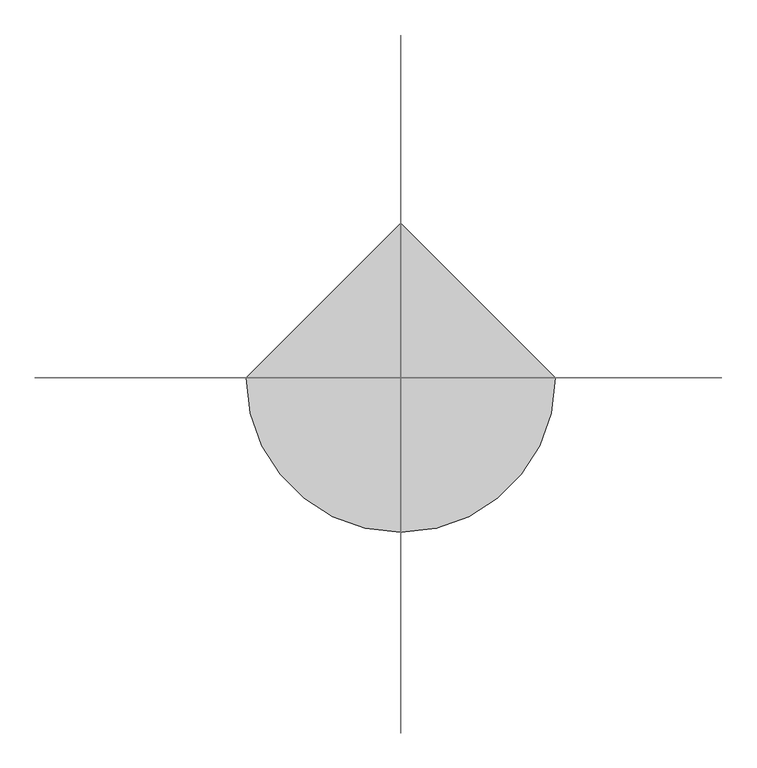
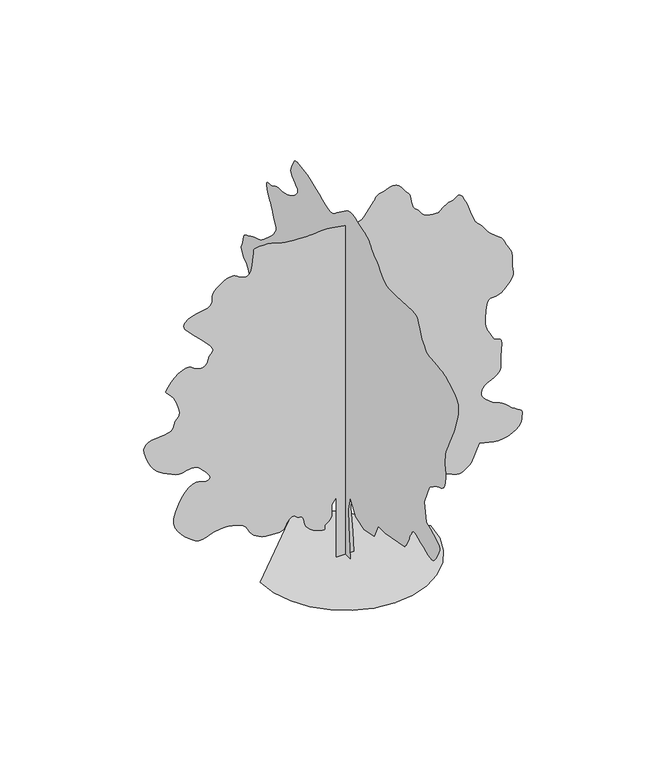
"""IFC4 building model written with IfcOpenShell, lengths in millimetres: geographic element geometry, RPC 木 - 落葉樹 : スカーレット オーク - 12.5 メートル."""

from ifc_helpers import new_model, si_unit, origin, place, context, project, spatial, triangles, source, transform, mapped, element, save


def geographic_element_78a4568a(model_context):
    return source(origin(), model_context, "Body", "Tessellation", [
        triangles([(0.0172504, 306.0074844, 0.0), (0.0172504, -293.5650026, 0.0), (0.0172504, -196.8600042, 1141.1200275), (0.0172504, -177.5185068, 1682.6674953), (0.0172504, -293.5650026, 2185.5350567), (0.0172504, -603.0224945, 1682.6674953), (0.0172504, -1105.8875124, 1527.9400211), (0.0172504, -1686.1174301, 1663.3275421), (0.0172504, -1918.2099495, 2146.8525341), (0.0172504, -2324.3725124, 2146.8525341), (0.0172504, -3446.150116, 2359.6049549), (0.0172504, -3487.4249222, 2409.394939), (0.0172504, -3527.7000801, 2459.5225479), (0.0172504, -3565.9250725, 2510.3249702), (0.0172504, -3601.0999603, 2562.1500046), (0.0172504, -3632.2250954, 2615.3249565), (0.0172504, -3658.2749588, 2670.2000954), (0.0172504, -3678.2499023, 2727.0751122), (0.0172504, -3697.649881, 2785.6750237), (0.0172504, -3722.1251312, 2845.2748741), (0.0172504, -3750.8251236, 2905.7249634), (0.0172504, -3782.89991, 2966.8500114), (0.0172504, -3817.5251221, 3028.475029), (0.0172504, -3853.8249413, 3090.4500252), (0.0172504, -3890.9999977, 3152.5750122), (0.0172504, -3908.7000801, 3172.6499496), (0.0172504, -3933.1750397, 3188.8501236), (0.0172504, -3971.1750458, 3197.2499016), (0.0172504, -4029.4749756, 3193.9751015), (0.0172504, -4114.8499969, 3175.1500877), (0.0172504, -4234.0499886, 3136.8500999), (0.0172504, -4393.8501183, 3075.2250824), (0.0172504, -4562.5749939, 3002.6998581), (0.0172504, -4706.2499451, 2937.9750298), (0.0172504, -4828.2750549, 2886.4249786), (0.0172504, -4932.0251175, 2853.4999535), (0.0172504, -5020.8999252, 2844.5999153), (0.0172504, -5098.249855, 2865.125116), (0.0172504, -5167.5002792, 2920.4999336), (0.0172504, -5237.3750839, 3007.7251328), (0.0172504, -5309.5997452, 3113.9000473), (0.0172504, -5377.1002762, 3229.5499649), (0.0172504, -5432.7497864, 3345.1998825), (0.0172504, -5469.4498718, 3451.3750877), (0.0172504, -5480.1248016, 3538.6249947), (0.0172504, -5457.6250122, 3597.424894), (0.0172504, -5402.6498795, 3641.7000984), (0.0172504, -5323.3000717, 3691.0249947), (0.0172504, -5223.6747574, 3744.5999222), (0.0172504, -5107.774855, 3801.5499344), (0.0172504, -4979.7251129, 3861.0500816), (0.0172504, -4843.5499947, 3922.2251266), (0.0172504, -4703.3251236, 3984.2501198), (0.0172504, -4587.2749397, 4641.8500969), (0.0172504, -4877.3749649, 5318.7747665), (0.0172504, -4886.5249878, 5331.7001404), (0.0172504, -4900.7252838, 5347.4747589), (0.0172504, -4925.0999588, 5369.0251877), (0.0172504, -4964.6748688, 5399.20009), (0.0172504, -5024.5502838, 5440.8498734), (0.0172504, -5109.8247299, 5496.8999405), (0.0172504, -5225.5252258, 5570.225116), (0.0172504, -5351.0501221, 5636.6501312), (0.0172504, -5462.3497238, 5680.0498077), (0.0172504, -5559.4501923, 5715.3499786), (0.0172504, -5642.3497833, 5757.424736), (0.0172504, -5711.0252426, 5821.1499161), (0.0172504, -5765.4998245, 5921.4001923), (0.0172504, -5805.7502747, 6073.0752365), (0.0172504, -5829.0500153, 6222.0498642), (0.0172504, -5835.7501877, 6317.5748474), (0.0172504, -5830.6249191, 6379.6001312), (0.0172504, -5818.3750854, 6428.1000778), (0.0172504, -5803.7748138, 6483.0252136), (0.0172504, -5791.5499786, 6564.3249023), (0.0172504, -5786.4247101, 6692.0002487), (0.0172504, -5788.2251816, 6832.849791), (0.0172504, -5796.1252808, 6949.6752182), (0.0172504, -5813.8247818, 7056.3751007), (0.0172504, -5845.0502014, 7166.7747574), (0.0172504, -5893.550148, 7294.7750839), (0.0172504, -5963.0249771, 7454.2502335), (0.0172504, -6057.1750443, 7659.049942), (0.0172504, -6146.5748199, 7844.1752701), (0.0172504, -6206.1752518, 7955.8748474), (0.0172504, -6246.4751175, 8024.9502823), (0.0172504, -6277.9999374, 8082.1752777), (0.0172504, -6311.225235, 8158.3502792), (0.0172504, -6356.599791, 8284.2751511), (0.0172504, -6424.6752869, 8490.6997604), (0.0172504, -6498.0248795, 8729.4997192), (0.0172504, -6547.3747742, 8935.1499573), (0.0172504, -6565.2498459, 9112.3751862), (0.0172504, -6544.199968, 9265.925116), (0.0172504, -6476.8250107, 9400.5250397), (0.0172504, -6355.6498489, 9520.9002502), (0.0172504, -6173.2249374, 9631.8248749), (0.0172504, -5996.2252762, 9723.0001236), (0.0172504, -5879.7998245, 9785.7747803), (0.0172504, -5799.2250916, 9827.2001587), (0.0172504, -5729.8002594, 9854.4496582), (0.0172504, -5646.85009, 9874.575174), (0.0172504, -5525.6749283, 9894.699527), (0.0172504, -5341.575119, 9921.9501892), (0.0172504, -5144.0999634, 9943.4244598), (0.0172504, -4990.9500092, 9951.725116), (0.0172504, -4869.5998581, 9962.0244873), (0.0172504, -4767.5499825, 9989.5995483), (0.0172504, -4672.2499855, 10049.6505341), (0.0172504, -4571.2000488, 10157.425351), (0.0172504, -4451.8750648, 10328.0998169), (0.0172504, -4347.6750298, 10515.7499908), (0.0172504, -4286.1000092, 10666.5500885), (0.0172504, -4245.8501404, 10783.8254883), (0.0172504, -4205.5749825, 10871.0003998), (0.0172504, -4143.9999619, 10931.4501984), (0.0172504, -4039.7999268, 10968.5502594), (0.0172504, -3871.650016, 10985.7003754), (0.0172504, -2943.2749969, 10927.6748474), (0.0172504, -2772.1499771, 10930.6746643), (0.0172504, -2632.8250511, 10930.2746887), (0.0172504, -2514.4500092, 10937.3254211), (0.0172504, -2406.244986, 10962.6250397), (0.0172504, -2297.3600624, 11017.0496246), (0.0172504, -2176.9724979, 11111.3752625), (0.0172504, -2034.2550465, 11256.4745453), (0.0172504, -1896.7275398, 11403.0249023), (0.0172504, -1793.7050491, 11502.8746216), (0.0172504, -1717.0749882, 11568.5752625), (0.0172504, -1658.7125622, 11612.6248993), (0.0172504, -1610.5025688, 11647.5250946), (0.0172504, -1564.320068, 11685.7995026), (0.0172504, -1512.0500027, 11739.9996826), (0.0172504, -1461.8649845, 11804.0004272), (0.0172504, -1420.8125484, 11863.6002777), (0.0172504, -1379.087479, 11919.1503754), (0.0172504, -1326.8724976, 11970.9495392), (0.0172504, -1254.3574471, 12019.4000702), (0.0172504, -1151.7299904, 12064.7996246), (0.0172504, -1009.182514, 12107.4749268), (0.0172504, -849.1549999, 12154.4999634), (0.0172504, -699.9524792, 12206.6002716), (0.0172504, -560.5600064, 12254.6496643), (0.0172504, -429.9675053, 12289.4998627), (0.0172504, -307.1550161, 12302.0246796), (0.0172504, -191.1079934, 12283.0746735), (0.0172504, -80.8134993, 12223.5248199), (0.0172504, 499.4175176, 11798.0252106), (0.0172504, 562.2325061, 11740.8496307), (0.0172504, 623.0199657, 11688.7504852), (0.0172504, 689.217524, 11646.7751404), (0.0172504, 768.2749804, 11620.0500275), (0.0172504, 867.630035, 11613.6248383), (0.0172504, 994.7275097, 11632.5748444), (0.0172504, 1157.0125168, 11681.9753174), (0.0172504, 1341.1749676, 11755.3254913), (0.0172504, 1526.6899521, 11837.8251068), (0.0172504, 1710.1749733, 11922.0246185), (0.0172504, 1888.2475342, 12000.4500641), (0.0172504, 2057.5249924, 12065.6995697), (0.0172504, 2214.6200546, 12110.3003357), (0.0172504, 2356.1550201, 12126.8249084), (0.0172504, 2484.8875694, 12135.849939), (0.0172504, 2604.4750374, 12156.3754303), (0.0172504, 2712.9251038, 12178.575238), (0.0172504, 2808.1501053, 12192.6755402), (0.0172504, 2888.1748718, 12188.8501923), (0.0172504, 2950.9251114, 12157.2753754), (0.0172504, 2994.400074, 12088.1249451), (0.0172504, 3033.2500282, 12001.2500153), (0.0172504, 3077.8499222, 11921.1246735), (0.0172504, 3119.7499809, 11845.0502472), (0.0172504, 3150.5001389, 11770.3245758), (0.0172504, 3161.6000427, 11694.2745667), (0.0172504, 3144.6249161, 11614.1503876), (0.0172504, 3091.124984, 11527.2498779), (0.0172504, 3009.2500397, 11447.6245056), (0.0172504, 2921.5998665, 11385.2504059), (0.0172504, 2841.4251091, 11331.3502075), (0.0172504, 2781.8749649, 11277.1000305), (0.0172504, 2756.1750801, 11213.7248291), (0.0172504, 2777.4749428, 11132.4251404), (0.0172504, 2859.0249069, 11024.3747589), (0.0172504, 2971.6250107, 10916.7255157), (0.0172504, 3077.7999252, 10838.2000763), (0.0172504, 3178.2249001, 10782.3), (0.0172504, 3273.574894, 10742.6745117), (0.0172504, 3364.5248657, 10712.8251709), (0.0172504, 3451.7750633, 10686.4000397), (0.0172504, 3535.9498672, 10656.8995148), (0.0172504, 3620.024968, 10634.1753204), (0.0172504, 3706.4749237, 10626.6746155), (0.0172504, 3795.2750267, 10625.9502411), (0.0172504, 3886.4499847, 10623.5248077), (0.0172504, 3980.0000885, 10610.9499939), (0.0172504, 4075.9250473, 10579.7495728), (0.0172504, 4174.1998627, 10521.5252197), (0.0172504, 4275.775058, 10469.80047), (0.0172504, 4375.6250679, 10451.2504395), (0.0172504, 4465.0001358, 10446.8995422), (0.0172504, 4535.0999268, 10437.8245148), (0.0172504, 4577.0999794, 10405.075351), (0.0172504, 4582.2249573, 10329.6753021), (0.0172504, 4541.7001053, 10192.7255219), (0.0172504, 4481.7999825, 10048.5994354), (0.0172504, 4432.0751106, 9951.4995483), (0.0172504, 4388.424868, 9882.1247131), (0.0172504, 4346.8250816, 9821.224942), (0.0172504, 4303.1751297, 9749.5002502), (0.0172504, 4253.4249687, 9647.6750702), (0.0172504, 4193.550135, 9496.4499985), (0.0172504, 4130.2749275, 9347.6997757), (0.0172504, 4075.8250534, 9253.7502777), (0.0172504, 4034.1999779, 9195.999733), (0.0172504, 4009.500032, 9155.8498581), (0.0172504, 4005.7749687, 9114.7000443), (0.0172504, 4027.1001205, 9053.900267), (0.0172504, 4077.4999512, 8954.8999146), (0.0172504, 4167.2249977, 8823.6747849), (0.0172504, 4293.1248711, 8684.3501495), (0.0172504, 4439.3499573, 8545.349913), (0.0172504, 4589.9500671, 8415.1497208), (0.0172504, 4729.0750053, 8302.2002197), (0.0172504, 4840.7748734, 8214.9747299), (0.0172504, 4909.1747681, 8161.9000626), (0.0172504, 4969.9001312, 8128.6997635), (0.0172504, 5061.0747986, 8095.1500671), (0.0172504, 5170.5250946, 8060.9248306), (0.0172504, 5286.0750183, 8025.675238), (0.0172504, 5395.524733, 7989.0751465), (0.0172504, 5486.6999817, 7950.8001572), (0.0172504, 5547.4247635, 7910.4747116), (0.0172504, 5598.275148, 7876.9750122), (0.0172504, 5663.0252655, 7853.2997131), (0.0172504, 5734.1749924, 7830.2999542), (0.0172504, 5804.3247803, 7798.8251312), (0.0172504, 5866.0250839, 7749.7752182), (0.0172504, 5911.8001968, 7673.9751938), (0.0172504, 5934.2499893, 7562.325032), (0.0172504, 5952.6250305, 7450.1749008), (0.0172504, 5984.1998474, 7370.8500916), (0.0172504, 6018.4750809, 7312.1501862), (0.0172504, 6045.000206, 7261.899765), (0.0172504, 6053.2252853, 7207.9501511), (0.0172504, 6032.699794, 7138.074765), (0.0172504, 5972.9249542, 7040.1249298), (0.0172504, 5898.7248322, 6948.3747162), (0.0172504, 5838.7250061, 6893.5251572), (0.0172504, 5788.2001831, 6857.9500031), (0.0172504, 5742.4000717, 6824.0497467), (0.0172504, 5696.6249588, 6774.2498795), (0.0172504, 5646.1001358, 6690.9747299), (0.0172504, 5586.0997284, 6556.5997925), (0.0172504, 5520.7002319, 6421.9998688), (0.0172504, 5460.6998245, 6337.1498154), (0.0172504, 5411.5249191, 6283.075209), (0.0172504, 5378.6001846, 6240.824881), (0.0172504, 5367.3247101, 6191.4999847), (0.0172504, 5383.09991, 6116.0999359), (0.0172504, 5431.3748703, 5995.7247253), (0.0172504, 5495.5000259, 5864.0502045), (0.0172504, 5555.8748291, 5761.8250488), (0.0172504, 5613.5747955, 5680.5747757), (0.0172504, 5669.5498672, 5611.8249023), (0.0172504, 5724.8749786, 5547.1497803), (0.0172504, 5780.5250702, 5478.0749268), (0.0172504, 5837.5250793, 5396.1502762), (0.0172504, 5903.6751114, 5315.3499756), (0.0172504, 5980.6500641, 5249.4249298), (0.0172504, 6060.324852, 5189.6000931), (0.0172504, 6134.5999695, 5127.0498413), (0.0172504, 6195.3247513, 5053.0252899), (0.0172504, 6234.4002731, 4958.675235), (0.0172504, 6243.7002869, 4835.2499199), (0.0172504, 6251.5248093, 4738.3250221), (0.0172504, 6280.349794, 4706.349939), (0.0172504, 6313.2251129, 4704.825032), (0.0172504, 6333.2500534, 4699.2500816), (0.0172504, 6323.4750687, 4655.0998695), (0.0172504, 6267.0500244, 4537.8750481), (0.0172504, 6146.999794, 4313.0501083), (0.0172504, 6021.4748978, 4060.8750938), (0.0172504, 5945.6998718, 3875.3750793), (0.0172504, 5898.3248566, 3742.6250427), (0.0172504, 5858.0749878, 3648.7999557), (0.0172504, 5803.5998245, 3580.0000854), (0.0172504, 5713.6000854, 3522.3751144), (0.0172504, 5566.7747452, 3462.0500175), (0.0172504, 5397.250209, 3413.1000984), (0.0172504, 5248.0500137, 3392.5748978), (0.0172504, 5111.025238, 3390.9999939), (0.0172504, 4978.0752136, 3398.9000931), (0.0172504, 4841.0498566, 3406.7749031), (0.0172504, 4691.8499519, 3405.1999992), (0.0172504, 4522.3501236, 3384.6750893), (0.0172504, 4353.2999771, 3366.3000481), (0.0172504, 4207.2498802, 3370.2500977), (0.0172504, 4078.7998718, 3385.7000267), (0.0172504, 3962.5249924, 3401.8249146), (0.0172504, 3853.0249901, 3407.8001312), (0.0172504, 3744.8749054, 3392.799884), (0.0172504, 3632.6500694, 3346.0001244), (0.0172504, 3525.249939, 3296.2499634), (0.0172504, 3436.4251282, 3270.2000999), (0.0172504, 3368.249929, 3253.6249489), (0.0172504, 3322.75009, 3232.3250862), (0.0172504, 3301.9499062, 3192.0499283), (0.0172504, 3307.8751259, 3118.6500481), (0.0172504, 3342.5500443, 2997.8498634), (0.0172504, 3398.475119, 2869.5251381), (0.0172504, 3465.5750931, 2778.7248665), (0.0172504, 3542.0000793, 2719.2500084), (0.0172504, 3625.8499031, 2684.8000763), (0.0172504, 3715.274968, 2669.1248703), (0.0172504, 3808.4250961, 2665.9500641), (0.0172504, 3903.4251114, 2669.0498749), (0.0172504, 4270.9250633, 2262.8999565), (0.0172504, 4299.7250496, 2217.1674282), (0.0172504, 4327.3501076, 2170.5925095), (0.0172504, 4352.6250183, 2122.3249615), (0.0172504, 4374.3248566, 2071.5174522), (0.0172504, 4391.2999832, 2017.3300621), (0.0172504, 4402.3498901, 1958.9125523), (0.0172504, 4406.2999397, 1895.4200615), (0.0172504, 4405.6249809, 1829.2200325), (0.0172504, 4400.8999786, 1763.6974331), (0.0172504, 4388.0248924, 1699.5299835), (0.0172504, 4362.9999664, 1637.3900265), (0.0172504, 4321.7248695, 1577.9574623), (0.0172504, 4260.1501396, 1521.9075405), (0.0172504, 4174.1998627, 1469.9175453), (0.0172504, 4092.2249245, 1425.7650078), (0.0172504, 4034.5999535, 1391.4249527), (0.0172504, 3985.4250481, 1364.8675621), (0.0172504, 3928.800016, 1344.0599659), (0.0172504, 3848.8499542, 1326.9749622), (0.0172504, 3729.6499626, 1311.5799717), (0.0172504, 3555.3001396, 1295.8475018), (0.0172504, 3356.9750359, 1298.1024513), (0.0172504, 3174.2251442, 1332.8375404), (0.0172504, 3003.6500908, 1392.27243), (0.0172504, 2841.8750816, 1468.6199501), (0.0172504, 2685.525032, 1554.1049938), (0.0172504, 2531.1748604, 1640.9425713), (0.0172504, 2375.4949734, 1721.3500179), (0.0172504, 2236.6675461, 1794.4849434), (0.0172504, 2129.3050587, 1863.5599422), (0.0172504, 2044.6099377, 1926.8850014), (0.0172504, 1973.7875164, 1982.7650208), (0.0172504, 1908.0399307, 2029.5099873), (0.0172504, 1838.5700432, 2065.4300331), (0.0172504, 1756.5824604, 2088.8300583), (0.0172504, 1666.4174698, 2108.5650455), (0.0172504, 1577.6074837, 2133.0375343), (0.0172504, 1489.134977, 2159.8799366), (0.0172504, 1399.9875114, 2186.7200134), (0.0172504, 1309.1449459, 2211.1925022), (0.0172504, 1215.5975309, 2230.9274895), (0.0172504, 1118.3299942, 2243.5575325), (0.0172504, 1018.8625191, 2250.1549496), (0.0172504, 919.3925005, 2253.7074944), (0.0172504, 819.9250254, 2254.7225487), (0.0172504, 720.4574776, 2253.7074944), (0.0172504, 620.9900024, 2251.1700039), (0.0172504, 521.5199839, 2247.6174591), (0.0172504, 422.0525087, 2243.5575325), (0.0172504, 228.6430025, 1953.4425373), (0.0172504, 189.960498, 1508.6000679), (280.4450004, 0.0006008, 0.0092122), (-299.7850081, 0.0006008, 0.0092122), (-299.7850081, 0.0004756, 2127.5199932), (-454.5149895, 0.0004756, 1914.7700432), (-454.5149895, 0.0005007, 1682.6775238), (-450.9625174, 0.0005007, 1628.8274677), (-450.9625174, 0.0005007, 1575.1449886), (-458.0674979, 0.0005007, 1521.8024597), (-475.8274967, 0.0005257, 1468.967458), (-507.8000001, 0.0005257, 1416.8100311), (-557.5350094, 0.0005257, 1365.4949947), (-628.5824896, 0.0005257, 1315.1974834), (-684.2375227, 0.0005257, 1262.982502), (-699.6325132, 0.0005257, 1210.0900183), (-696.0799685, 0.0005257, 1162.9524885), (-694.8950117, 0.0005257, 1127.990015), (-717.3950191, 0.0005257, 1111.6375248), (-784.8900272, 0.0005257, 1120.3225325), (-918.6974848, 0.0005257, 1160.4700092), (-1071.3399845, 0.0005257, 1223.0050003), (-1185.4125275, 0.0005257, 1293.6575191), (-1267.3425556, 0.0005257, 1371.0799736), (-1323.5625252, 0.0005257, 1453.9125629), (-1360.49748, 0.0005007, 1540.8049335), (-1384.5749348, 0.0005007, 1630.4049877), (-1402.2250202, 0.0005007, 1721.3600464), (-1406.7350647, 0.0005007, 1746.1124599), (-1413.4449749, 0.0005007, 1770.19006), (-1424.5524364, 0.0005007, 1792.9174519), (-1442.2599312, 0.0005007, 1813.6099388), (-1468.7600578, 0.0005007, 1831.5975037), (-1506.2599491, 0.0005007, 1846.2025715), (-1556.9524944, 0.0005007, 1856.7475674), (-1607.6450397, 0.0005007, 1874.1124958), (-1647.5100483, 0.0005007, 1903.3224861), (-1682.3025467, 0.0004756, 1934.9000645), (-1717.7700039, 0.0004756, 1959.3725533), (-1759.6674465, 0.0004756, 1967.2675655), (-1813.7424889, 0.0004756, 1949.1099529), (-1885.7500122, 0.0005007, 1895.4274738), (-1949.0724552, 0.0005007, 1820.3199944), (-1984.9925011, 0.0005007, 1746.902528), (-2011.1000645, 0.0005007, 1679.2374722), (-2044.9875309, 0.0005007, 1621.382428), (-2104.2525181, 0.0005007, 1577.4025543), (-2206.4824699, 0.0005007, 1551.3499294), (-2369.2750042, 0.0005007, 1547.2900028), (-2549.149926, 0.0005007, 1559.2449417), (-2695.2000229, 0.0005007, 1578.979929), (-2813.8250496, 0.0005007, 1607.1750103), (-2911.4999016, 0.0005007, 1644.5025284), (-2994.6250603, 0.0005007, 1691.6425289), (-3069.600135, 0.0005007, 1749.2724415), (-3142.9250198, 0.0005007, 1818.0650448), (-3205.1000038, 0.0005007, 1893.5100037), (-3249.7248962, 0.0004756, 1969.2975288), (-3287.549913, 0.0004756, 2043.389954), (-3329.4499718, 0.0004756, 2113.7625481), (-3386.2249947, 0.0004756, 2178.3824409), (-3468.7249008, 0.0004756, 2235.2224308), (-3587.7499031, 0.0004756, 2282.2499382), (-3707.4248657, 0.0004756, 2317.9974655), (-3794.2500893, 0.0004506, 2343.2600224), (-3862.8249733, 0.0004506, 2359.3875263), (-3927.6750847, 0.0004506, 2367.7325111), (-4003.3251183, 0.0004506, 2369.6499813), (-4104.3750549, 0.0004506, 2366.4924706), (-4245.3498802, 0.0004506, 2359.6125126), (-4400.3500122, 0.0004506, 2335.1974331), (-4538.1250328, 0.0004756, 2289.8050003), (-4665.0501343, 0.0004756, 2240.3524956), (-4787.5749229, 0.0004756, 2203.7574909), (-4912.1501678, 0.0004756, 2196.9349422), (-5045.1501892, 0.0004756, 2236.7999508), (-5193.0498825, 0.0004506, 2340.2725594), (-5347.7997391, 0.0004506, 2478.6475433), (-5490.6747391, 0.0004506, 2615.9999153), (-5612.2498764, 0.0004256, 2758.4499413), (-5703.0251495, 0.0004256, 2912.049868), (-5753.5499725, 0.0004256, 3082.8999046), (-5754.3499237, 0.0004005, 3277.0999695), (-5695.9250015, 0.0004005, 3500.7249825), (-5598.1501556, 0.0003755, 3726.2748779), (-5489.1998291, 0.0003755, 3919.6999901), (-5372.1499969, 0.0003505, 4077.2499664), (-5250.0248932, 0.0003505, 4195.2000343), (-5125.8499146, 0.0003505, 4269.8501289), (-5002.6998734, 0.0003505, 4297.4998947), (-4883.6001663, 0.0003505, 4274.3751434), (-4771.2750458, 0.0003505, 4235.4749016), (-4671.8250114, 0.0003505, 4218.8750427), (-4593.3248611, 0.0003505, 4225.6499199), (-4543.9249695, 0.0003505, 4256.7750549), (-4531.7501312, 0.0003505, 4313.2750946), (-4564.9001427, 0.0003505, 4396.1749763), (-4651.5000893, 0.0003254, 4506.4749298), (-4752.500029, 0.0003254, 4617.0998634), (-4829.4749817, 0.0003254, 4702.3498924), (-4891.5502625, 0.0003254, 4765.2751213), (-4947.8747314, 0.0003254, 4808.9250732), (-5007.6001556, 0.0003254, 4836.325145), (-5079.8248169, 0.0003004, 4850.5498581), (-5173.7248993, 0.0003004, 4854.5999016), (-5270.0248352, 0.0003254, 4845.5248741), (-5349.7751999, 0.0003254, 4824.5999886), (-5422.3998367, 0.0003254, 4801.3249557), (-5497.39991, 0.0003254, 4785.1250725), (-5584.2248428, 0.0003254, 4785.5250481), (-5692.3752182, 0.0003254, 4811.9748871), (-5831.3248764, 0.0003004, 4873.9498833), (-5978.7751785, 0.0003004, 4948.0997177), (-6108.6248108, 0.0003004, 5012.4248611), (-6224.6252884, 0.0003004, 5078.4748993), (-6330.4502243, 0.0003004, 5157.6997147), (-6429.8749695, 0.0003004, 5261.5997681), (-6526.574881, 0.0002754, 5401.7249359), (-6624.2997299, 0.0002754, 5589.5750977), (-6705.1000305, 0.0002503, 5784.4998276), (-6749.7002151, 0.0002503, 5941.2001465), (-6759.8001801, 0.0002503, 6064.0752045), (-6737.074823, 0.0002253, 6157.4997345), (-6683.2252029, 0.0002253, 6225.9002106), (-6599.9500534, 0.0002253, 6273.6502029), (-6488.899855, 0.0002253, 6305.1750229), (-6357.7997177, 0.0002253, 6323.2750809), (-6219.2750336, 0.0002253, 6333.9500107), (-6082.4002487, 0.0002253, 6346.2748398), (-5956.3748016, 0.0002253, 6369.4501694), (-5850.3248795, 0.0002253, 6412.5998611), (-5773.3499268, 0.0002253, 6484.8251038), (-5734.5999664, 0.0002003, 6595.2997559), (-5705.9749695, 0.0002003, 6701.9752213), (-5661.749762, 0.0002003, 6771.4500504), (-5614.8497177, 0.0002003, 6825.7002274), (-5578.0752182, 0.0002003, 6886.6999924), (-5564.3248947, 0.0001752, 6976.4747452), (-5586.4252899, 0.0001752, 7116.9998886), (-5657.2500366, 0.0001752, 7330.2502441), (-5757.5497284, 0.0001502, 7540.3002136), (-5853.4752686, 0.0001502, 7672.5252823), (-5935.8498917, 0.0001502, 7750.975145), (-5995.5747345, 0.0001252, 7799.6250824), (-6023.4747757, 0.0001252, 7842.5247894), (-6010.4499893, 0.0001252, 7903.7251236), (-5947.3497711, 0.0001252, 8007.2002029), (-5845.6501648, 0.0001252, 8136.3248795), (-5728.0247864, 0.0001001, 8253.9502579), (-5602.2749039, 0.0001001, 8353.3000076), (-5476.1750427, 0.0001001, 8427.6251221), (-5357.5497253, 0.0001001, 8470.1248535), (-5254.1252243, 0.0001001, 8474.0751938), (-5173.7248993, 0.0001001, 8432.6998123), (-5094.9000595, 0.0001001, 8371.00009), (-4997.8001724, 0.0001001, 8322.8501221), (-4892.5751999, 0.0001001, 8294.6500992), (-4789.3751038, 0.0001001, 8292.850209), (-4698.375135, 0.0001001, 8323.8750595), (-4629.6999664, 0.0001001, 8394.1248413), (-4593.5001411, 0.0001001, 8510.0497421), (-4560.3251312, 0.0001001, 8620.5749725), (-4508.2251137, 7.51e-05, 8686.1000427), (-4458.4999512, 7.51e-05, 8730.3002518), (-4432.4500877, 7.51e-05, 8776.8747345), (-4451.4000938, 7.51e-05, 8849.4999527), (-4536.6501228, 7.51e-05, 8971.8750412), (-4709.5500343, 5.01e-05, 9167.6497192), (-4926.3498825, 5.01e-05, 9388.800174), (-5120.1502625, 2.5e-05, 9575.0998489), (-5277.4249649, 2.5e-05, 9731.9751572), (-5384.5998184, 2.5e-05, 9864.8246063), (-5428.2000641, 0.0, 9979.0746094), (-5394.6497864, 0.0, 10080.1254181), (-5270.4248108, 0.0, 10173.3755402), (-5104.7500397, 0.0, 10245.2246429), (-4956.3497955, 0.0, 10286.2744629), (-4825.8749107, 0.0, 10308.3754395), (-4714.0000534, -2.5e-05, 10323.3745239), (-4621.3998917, -2.5e-05, 10343.1000641), (-4548.7749641, -2.5e-05, 10379.4245911), (-4496.7749405, -2.5e-05, 10444.1497101), (-4470.8500694, -2.5e-05, 10520.7252686), (-4466.9000198, -2.5e-05, 10587.8246613), (-4471.4000359, -2.5e-05, 10650.1999237), (-4470.8500694, -2.5e-05, 10712.5751862), (-4451.6750771, -5.01e-05, 10779.6745789), (-4400.3500122, -5.01e-05, 10856.2501373), (-4303.3751175, -5.01e-05, 10947.0248291), (-4184.6750954, -5.01e-05, 11036.8495789), (-4076.1250351, -5.01e-05, 11106.7255463), (-3976.0500389, -7.51e-05, 11155.60047), (-3882.7249214, -7.51e-05, 11182.4999908), (-3794.4750755, -7.51e-05, 11186.3997528), (-3709.6000237, -7.51e-05, 11166.2498199), (-3626.4498665, -5.01e-05, 11121.1002502), (-3540.7248665, -5.01e-05, 11065.9001312), (-3452.3250298, -5.01e-05, 11022.8748505), (-3365.6000908, -5.01e-05, 11001.8249725), (-3284.9500717, -5.01e-05, 11012.5998962), (-3214.7999931, -5.01e-05, 11064.9746063), (-3159.5498772, -7.51e-05, 11168.7996643), (-3123.5750381, -7.51e-05, 11333.8500549), (-3102.0998955, -7.51e-05, 11511.0752838), (-3086.6999634, -0.0001001, 11648.0250641), (-3076.3750122, -0.0001001, 11749.4746857), (-3070.125103, -0.0001001, 11820.1250244), (-3066.9000092, -0.0001001, 11864.7246277), (-3065.7250809, -0.0001001, 11888.025531), (-3065.5500916, -0.0001001, 11894.7251221), (-3040.1248993, -0.0001001, 11898.674881), (-2971.0500458, -0.0001001, 11907.3755127), (-2869.1498703, -0.0001001, 11916.0505646), (-2745.2748734, -0.0001001, 11920.0003235), (-2610.2249771, -0.0001001, 11914.4750793), (-2474.8323692, -0.0001001, 11894.7251221), (-2349.935051, -0.0001001, 11856.0495758), (-2235.4100647, -0.0001001, 11813.0254578), (-2120.5474537, -0.0001001, 11781.8494537), (-2000.2725277, -0.0001001, 11760.1251984), (-1869.5075443, -0.0001001, 11745.5249268), (-1723.1824642, -0.0001001, 11735.675528), (-1556.2175102, -0.0001001, 11728.174823), (-1363.5400269, -0.0001001, 11720.6752808), (-1177.5749971, -0.0001001, 11719.599765), (-1024.4249702, -0.0001001, 11728.6747925), (-889.5449764, -0.0001001, 11741.475174), (-758.3875025, -0.0001001, 11751.5745575), (-616.4050352, -0.0001001, 11752.5244995), (-449.0450109, -0.0001001, 11737.9253906), (-241.763259, -0.0001001, 11701.3252991), (-32.2257492, -0.0001001, 11657.8000488), (136.7125037, -0.0001001, 11627.7995544), (271.8174929, -0.0001001, 11613.0248749), (379.8574825, -0.0001001, 11615.1503265), (467.5975121, -0.0001001, 11635.9246399), (541.8025031, -0.0001001, 11676.9744598), (609.2425, -0.0001001, 11739.9996826), (899.3575315, -0.0001252, 12107.4749268), (942.8899761, -0.0001252, 12164.1505371), (977.6249926, -0.0001252, 12217.4496094), (1008.9749685, -0.0001252, 12266.3245331), (1042.3575239, -0.0001252, 12309.7997864), (1083.1825029, -0.0001252, 12346.8498505), (1136.864982, -0.0001252, 12376.4503693), (1208.8150234, -0.0001252, 12397.6002411), (1297.0049892, -0.0001502, 12421.8499237), (1393.3149536, -0.0001502, 12454.2246918), (1494.0224693, -0.0001502, 12483.8752075), (1595.4100307, -0.0001502, 12499.9998047), (1693.7499584, -0.0001502, 12491.7747253), (1785.3225666, -0.0001502, 12448.349469), (1866.410059, -0.0001252, 12358.9246948), (1938.4149662, -0.0001252, 12256.9251068), (2004.3324543, -0.0001252, 12177.5752991), (2062.8075188, -0.0001252, 12112.7746033), (2112.4850098, -0.0001252, 12054.4246765), (2152.0125389, -0.0001252, 11994.3748535), (2180.0375725, -0.0001001, 11924.5000488), (2195.2049606, -0.0001001, 11836.6995941), (2205.7499565, -0.0001001, 11745.7004974), (2220.3550243, -0.0001001, 11669.9248901), (2238.3424438, -0.0001001, 11606.8252533), (2259.0349308, -7.51e-05, 11553.8749969), (2281.7599972, -7.51e-05, 11508.5254395), (2305.8374519, -7.51e-05, 11468.2755707), (2330.5924816, -7.51e-05, 11430.5499664), (2355.6274361, -7.51e-05, 11413.5754211), (2381.680061, -7.51e-05, 11394.2254395), (2409.760033, -7.51e-05, 11370.1501648), (2440.8876389, -7.51e-05, 11338.9753235), (2476.0724098, -7.51e-05, 11298.3254791), (2516.3248947, -7.51e-05, 11245.8251953), (2562.6749725, -7.51e-05, 11179.1246155), (2631.3751396, -5.01e-05, 11115.7249969), (2728.4750267, -5.01e-05, 11072.3253204), (2839.7749191, -5.01e-05, 11045.1246552), (2951.0751022, -5.01e-05, 11030.4755493), (3048.1749893, -5.01e-05, 11024.6003265), (3116.8748657, -5.01e-05, 11023.8247925), (3142.9250198, -5.01e-05, 11024.4003387), (3156.2750771, -5.01e-05, 11038.3250702), (3192.9998703, -5.01e-05, 11074.2252045), (3247.9750031, -5.01e-05, 11123.3501129), (3316.1499115, -7.51e-05, 11176.8503357), (3392.4249069, -7.51e-05, 11225.9752441), (3471.7750053, -7.51e-05, 11261.8997955), (3549.0749382, -7.51e-05, 11275.824527), (3618.3750687, -7.51e-05, 11292.800235), (3679.5501137, -7.51e-05, 11331.0746429), (3736.350135, -7.51e-05, 11371.7244873), (3792.4499084, -7.51e-05, 11395.8253418), (3851.6000771, -7.51e-05, 11384.3748779), (3917.5251228, -7.51e-05, 11318.4498322), (3993.9251106, -7.51e-05, 11179.1246155), (4065.8750793, -5.01e-05, 11015.4253052), (4119.5500008, -5.01e-05, 10883.1996552), (4160.3751251, -5.01e-05, 10773.6249481), (4193.7501228, -2.5e-05, 10677.9505554), (4225.0999535, -2.5e-05, 10587.3246918), (4259.8498672, -2.5e-05, 10493.0002167), (4303.3751175, -2.5e-05, 10386.1253448), (4348.1000038, 0.0, 10292.3496735), (4386.3749931, 0.0, 10232.749823), (4423.6500435, 0.0, 10191.7755798), (4465.325116, 0.0, 10153.8255707), (4516.799881, 0.0, 10103.3495819), (4583.4998795, 0.0, 10024.7997253), (4670.850071, 0.0, 9902.6002075), (4778.3749031, 2.5e-05, 9766.6003693), (4896.3999664, 2.5e-05, 9652.9247498), (5016.4501968, 2.5e-05, 9555.474884), (5130.075238, 5.01e-05, 9468.1999786), (5228.8000259, 5.01e-05, 9384.974826), (5304.2000748, 5.01e-05, 9299.6997986), (5347.7997391, 5.01e-05, 9206.3252655), (5382.0249756, 5.01e-05, 9114.7500412), (5429.774968, 7.51e-05, 9032.6498199), (5483.3001892, 7.51e-05, 8950.5501801), (5534.7749542, 7.51e-05, 8858.9749557), (5576.449736, 7.51e-05, 8748.4747238), (5600.5250107, 0.0001001, 8609.5250656), (5599.22509, 0.0001001, 8432.6998123), (5596.5752518, 0.0001001, 8262.7497208), (5611.174942, 0.0001252, 8138.7997284), (5627.1251312, 0.0001252, 8042.949765), (5628.5500443, 0.0001252, 7957.224765), (5599.5000732, 0.0001252, 7863.750238), (5524.1250229, 0.0001502, 7744.5249573), (5386.4752853, 0.0001502, 7581.6750137), (5223.124791, 0.0001502, 7444.9502197), (5081.4247192, 0.0001502, 7390.0750809), (4961.7000504, 0.0001502, 7378.1752258), (4864.3248894, 0.0001502, 7370.3501221), (4789.60009, 0.0001752, 7327.6498215), (4737.9000481, 0.0001752, 7211.2249512), (4709.5250359, 0.0001752, 6982.1249817), (4698.9251015, 0.0002003, 6728.5997589), (4700.5250038, 0.0002003, 6550.1751846), (4714.6000168, 0.0002253, 6424.9002731), (4741.5751144, 0.0002253, 6330.7252075), (4781.7249893, 0.0002253, 6245.7001648), (4835.3999107, 0.0002253, 6147.7997452), (4902.950148, 0.0002503, 6015.0752884), (4980.0250946, 0.0002503, 5899.6497757), (5057.7999985, 0.0002503, 5847.1500732), (5129.8002548, 0.0002503, 5825.7752151), (5189.6250916, 0.0002503, 5803.7248169), (5230.8499008, 0.0002503, 5749.200238), (5247.0250763, 0.0002754, 5630.3749329), (5231.7498459, 0.0002754, 5415.5002579), (5210.9999496, 0.0003004, 5178.6001831), (5207.8251434, 0.0003004, 5005.3247131), (5211.4499222, 0.0003004, 4881.0997375), (5210.9999496, 0.0003254, 4791.3999802), (5195.6497238, 0.0003254, 4721.6498772), (5154.5999039, 0.0003254, 4657.3000259), (5077.0249878, 0.0003254, 4583.8248596), (4983.2998947, 0.0003254, 4514.9249954), (4900.3997223, 0.0003254, 4468.3499313), (4827.3251129, 0.0003254, 4435.6498924), (4763.0499664, 0.0003505, 4408.3501053), (4706.5499268, 0.0003505, 4378.0249214), (4656.8250549, 0.0003505, 4336.1748596), (4612.8251244, 0.0003505, 4274.3751434), (4577.8749321, 0.0003505, 4202.8248596), (4558.1249748, 0.0003505, 4135.32491), (4557.0000435, 0.0003505, 4068.8498978), (4577.8749321, 0.0003755, 4000.3250107), (4624.1000175, 0.0003755, 3926.7501411), (4699.1000908, 0.0003755, 3845.024897), (4806.2499458, 0.0003755, 3752.1750412), (4919.8002823, 0.0003755, 3670.8000664), (5016.1252167, 0.0003755, 3617.5001221), (5101.6002319, 0.0004005, 3580.1250778), (5182.6999329, 0.0004005, 3546.4750969), (5265.8000931, 0.0004005, 3504.3500519), (5357.374736, 0.0004005, 3441.5751045), (5463.8252151, 0.0004005, 3346.0001244), (5576.8497116, 0.0004005, 3247.2750458), (5681.0497467, 0.0004005, 3176.6249977), (5772.3999847, 0.0004256, 3124.2249985), (5846.8250931, 0.0004256, 3080.3000633), (5900.2747375, 0.0004256, 3035.0249199), (5928.6997467, 0.0004256, 2978.5748772), (5928.0247879, 0.0004256, 2901.1499519), (5916.924884, 0.0004256, 2813.2500847), (5910.1997131, 0.0004506, 2730.7498878), (5898.0748718, 0.0004506, 2651.975045), (5870.7247971, 0.0004506, 2575.2500771), (5818.350087, 0.0004506, 2498.8349739), (5731.1251785, 0.0004506, 2421.0750401), (5599.22509, 0.0004506, 2340.2725594), (5441.7248199, 0.0004756, 2274.8624531), (5284.2501297, 0.0004756, 2240.917432), (5126.7498596, 0.0004756, 2233.1924675), (4969.2501709, 0.0004756, 2246.4425308), (4811.7748993, 0.0004756, 2275.4250641), (4654.2749199, 0.0004756, 2314.8975094), (4496.7749405, 0.0004506, 2359.6125126), (4225.9998985, 0.0005007, 1760.042569), (4159.6498787, 0.0005007, 1702.5250042), (4092.9248817, 0.0005007, 1648.0549278), (4025.5499245, 0.0005007, 1599.675032), (3957.1500298, 0.0005007, 1560.4274277), (3887.3999268, 0.0005007, 1533.3625099), (3815.9499275, 0.0005007, 1521.5225349), (3742.4750519, 0.0005007, 1527.9500496), (3682.5999275, 0.0005007, 1542.5525013), (3644.6999153, 0.0005007, 1554.7899811), (3617.6501129, 0.0005007, 1567.0274609), (3590.2500412, 0.0005007, 1581.6300579), (3551.3250916, 0.0005007, 1600.9724819), (3489.750071, 0.0005007, 1627.4175247), (3394.3500801, 0.0005007, 1663.3375706), (3270.0751076, 0.0005007, 1715.4949974), (3134.2999649, 0.0005007, 1784.5699963), (2994.450071, 0.0005007, 1863.794957), (2857.9999695, 0.0004756, 1946.40256), (2732.3500809, 0.0004756, 2025.6275208), (2624.9999474, 0.0004756, 2094.7025196), (2543.3499893, 0.0004756, 2146.8625626), (2474.2126396, 0.0004756, 2192.817461), (2400.0074306, 0.0004756, 2246.8925034), (2321.5700672, 0.0004756, 2307.7374813), (2239.7525322, 0.0004506, 2373.9924488), (2155.3950359, 0.0004506, 2444.3074883), (2069.3475266, 0.0004506, 2517.3251244), (1982.4550106, 0.0004506, 2591.6999451), (1963.1124413, 0.0004256, 2881.8249687), (1576.2924477, 0.0004256, 2920.4999336), (880.0150349, 0.0004256, 2862.474987), (415.8325032, 0.0004506, 2611.0499268), (222.4215072, 0.0004756, 2146.8625626), (183.7397477, 0.0005007, 1605.3124786), (241.7622416, 0.0005507, 715.6274672), (-2855.9000977, 0.0, 0.0224297), (-2780.4000549, -654.3849844, 0.0224297), (-2565.3750984, -1255.3350037, 0.0224297), (-2228.0500488, -1785.6274899, 0.0224297), (-1785.6274899, -2228.0500488, 0.0224297), (-1255.3350037, -2565.3750984, 0.0224297), (-654.3849844, -2780.4000549, 0.0224297), (0.0001248, -2855.9000977, 0.0224297), (654.3849844, -2780.4000549, 0.0224297), (1255.3350037, -2565.3750984, 0.0224297), (1785.6274899, -2228.0500488, 0.0224297), (2228.0500488, -1785.6274899, 0.0224297), (2565.3750984, -1255.3350037, 0.0224297), (2780.4000549, -654.3849844, 0.0224297), (2855.9000977, 0.0002503, 0.0224297), (-0.0003745, 2855.9000977, 0.0224297)], [[1, 2, 3], [368, 1, 3], [368, 3, 4], [367, 368, 4], [367, 4, 5], [277, 278, 279], [366, 367, 5], [276, 277, 279], [276, 279, 280], [7, 8, 9], [6, 7, 9], [5, 6, 9], [315, 316, 317], [201, 202, 203], [200, 201, 203], [200, 203, 204], [199, 200, 204], [199, 204, 205], [198, 199, 205], [198, 205, 206], [198, 206, 207], [197, 198, 207], [197, 207, 208], [275, 276, 280], [196, 197, 208], [195, 196, 208], [194, 195, 208], [194, 208, 209], [193, 194, 209], [192, 193, 209], [192, 209, 210], [191, 192, 210], [191, 210, 211], [191, 211, 212], [190, 191, 212], [190, 212, 213], [190, 213, 214], [189, 190, 214], [189, 214, 215], [188, 189, 215], [187, 188, 215], [186, 187, 215], [10, 11, 12], [314, 315, 317], [10, 12, 13], [10, 13, 14], [10, 14, 15], [10, 15, 16], [10, 16, 17], [10, 17, 18], [10, 18, 19], [10, 19, 20], [10, 20, 21], [10, 21, 22], [185, 186, 215], [185, 215, 216], [275, 280, 281], [10, 22, 23], [167, 168, 169], [166, 167, 169], [165, 166, 169], [165, 169, 170], [164, 165, 170], [164, 170, 171], [163, 164, 171], [163, 171, 172], [163, 172, 173], [163, 173, 174], [163, 174, 175], [163, 175, 176], [163, 176, 177], [163, 177, 178], [163, 178, 179], [163, 179, 180], [162, 163, 180], [161, 162, 180], [160, 161, 180], [159, 160, 180], [159, 180, 181], [158, 159, 181], [157, 158, 181], [156, 157, 181], [156, 181, 182], [155, 156, 182], [154, 155, 182], [154, 182, 183], [9, 10, 23], [9, 23, 24], [9, 24, 25], [45, 46, 47], [44, 45, 47], [44, 47, 48], [43, 44, 48], [43, 48, 49], [42, 43, 49], [42, 49, 50], [41, 42, 50], [40, 41, 50], [40, 50, 51], [39, 40, 51], [38, 39, 51], [37, 38, 51], [36, 37, 51], [35, 36, 51], [34, 35, 51], [33, 34, 51], [33, 51, 52], [32, 33, 52], [32, 52, 53], [31, 32, 53], [30, 31, 53], [29, 30, 53], [28, 29, 53], [28, 53, 54], [27, 28, 54], [26, 27, 54], [5, 9, 25], [5, 25, 26], [5, 26, 54], [5, 54, 55], [366, 5, 55], [365, 366, 55], [364, 365, 55], [363, 364, 55], [362, 363, 55], [361, 362, 55], [361, 55, 56], [153, 154, 183], [153, 183, 184], [313, 314, 317], [360, 361, 56], [184, 185, 216], [153, 184, 216], [152, 153, 216], [152, 216, 217], [243, 244, 245], [242, 243, 245], [242, 245, 246], [241, 242, 246], [241, 246, 247], [241, 247, 248], [240, 241, 248], [240, 248, 249], [240, 249, 250], [239, 240, 250], [239, 250, 251], [238, 239, 251], [237, 238, 251], [236, 237, 251], [235, 236, 251], [234, 235, 251], [233, 234, 251], [232, 233, 251], [231, 232, 251], [230, 231, 251], [229, 230, 251], [228, 229, 251], [228, 251, 252], [227, 228, 252], [226, 227, 252], [226, 252, 253], [226, 253, 254], [226, 254, 255], [226, 255, 256], [226, 256, 257], [225, 226, 257], [224, 225, 257], [223, 224, 257], [222, 223, 257], [222, 257, 258], [221, 222, 258], [220, 221, 258], [115, 116, 117], [114, 115, 117], [114, 117, 118], [113, 114, 118], [113, 118, 119], [112, 113, 119], [111, 112, 119], [110, 111, 119], [152, 217, 218], [313, 317, 318], [313, 318, 319], [313, 319, 320], [313, 320, 321], [313, 321, 322], [313, 322, 323], [313, 323, 324], [313, 324, 325], [313, 325, 326], [313, 326, 327], [313, 327, 328], [313, 328, 329], [313, 329, 330], [313, 330, 331], [313, 331, 332], [313, 332, 333], [313, 333, 334], [313, 334, 335], [313, 335, 336], [313, 336, 337], [313, 337, 338], [313, 338, 339], [313, 339, 340], [313, 340, 341], [312, 313, 341], [312, 341, 342], [312, 342, 343], [311, 312, 343], [311, 343, 344], [311, 344, 345], [310, 311, 345], [310, 345, 346], [310, 346, 347], [310, 347, 348], [309, 310, 348], [309, 348, 349], [309, 349, 350], [308, 309, 350], [308, 350, 351], [307, 308, 351], [307, 351, 352], [307, 352, 353], [307, 353, 354], [307, 354, 355], [307, 355, 356], [307, 356, 357], [307, 357, 358], [306, 307, 358], [306, 358, 359], [306, 359, 360], [306, 360, 56], [305, 306, 56], [305, 56, 57], [304, 305, 57], [303, 304, 57], [302, 303, 57], [301, 302, 57], [301, 57, 58], [301, 58, 59], [110, 119, 120], [109, 110, 120], [109, 120, 121], [301, 59, 60], [300, 301, 60], [300, 60, 61], [151, 152, 218], [109, 121, 122], [300, 61, 62], [145, 146, 147], [144, 145, 147], [143, 144, 147], [143, 147, 148], [142, 143, 148], [141, 142, 148], [140, 141, 148], [140, 148, 149], [139, 140, 149], [138, 139, 149], [137, 138, 149], [136, 137, 149], [135, 136, 149], [134, 135, 149], [133, 134, 149], [132, 133, 149], [132, 149, 150], [131, 132, 150], [130, 131, 150], [129, 130, 150], [128, 129, 150], [127, 128, 150], [126, 127, 150], [126, 150, 151], [126, 151, 218], [125, 126, 218], [124, 125, 218], [123, 124, 218], [123, 218, 219], [122, 123, 219], [109, 122, 219], [108, 109, 219], [108, 219, 220], [108, 220, 258], [108, 258, 259], [108, 259, 260], [108, 260, 261], [108, 261, 262], [107, 108, 262], [107, 262, 263], [107, 263, 264], [106, 107, 264], [106, 264, 265], [106, 265, 266], [106, 266, 267], [106, 267, 268], [105, 106, 268], [104, 105, 268], [103, 104, 268], [102, 103, 268], [101, 102, 268], [100, 101, 268], [99, 100, 268], [98, 99, 268], [97, 98, 268], [96, 97, 268], [95, 96, 268], [94, 95, 268], [93, 94, 268], [92, 93, 268], [91, 92, 268], [90, 91, 268], [89, 90, 268], [88, 89, 268], [87, 88, 268], [86, 87, 268], [85, 86, 268], [84, 85, 268], [83, 84, 268], [82, 83, 268], [81, 82, 268], [80, 81, 268], [79, 80, 268], [78, 79, 268], [77, 78, 268], [76, 77, 268], [75, 76, 268], [74, 75, 268], [73, 74, 268], [72, 73, 268], [71, 72, 268], [70, 71, 268], [69, 70, 268], [68, 69, 268], [67, 68, 268], [66, 67, 268], [65, 66, 268], [64, 65, 268], [63, 64, 268], [62, 63, 268], [300, 62, 268], [299, 300, 268], [298, 299, 268], [297, 298, 268], [296, 297, 268], [295, 296, 268], [294, 295, 268], [293, 294, 268], [292, 293, 268], [291, 292, 268], [290, 291, 268], [289, 290, 268], [288, 289, 268], [287, 288, 268], [286, 287, 268], [285, 286, 268], [284, 285, 268], [283, 284, 268], [282, 283, 268], [281, 282, 268], [275, 281, 268], [275, 268, 269], [274, 275, 269], [274, 269, 270], [274, 270, 271], [273, 274, 271], [272, 273, 271], [802, 369, 370], [802, 370, 371], [801, 802, 371], [800, 801, 371], [575, 576, 577], [799, 800, 371], [574, 575, 577], [383, 384, 385], [383, 385, 386], [382, 383, 386], [382, 386, 387], [381, 382, 387], [381, 387, 388], [794, 795, 796], [510, 511, 512], [574, 577, 578], [573, 574, 578], [572, 573, 578], [572, 578, 579], [571, 572, 579], [571, 579, 580], [570, 571, 580], [570, 580, 581], [570, 581, 582], [569, 570, 582], [569, 582, 583], [569, 583, 584], [568, 569, 584], [568, 584, 585], [509, 510, 512], [509, 512, 513], [508, 509, 513], [508, 513, 514], [508, 514, 515], [507, 508, 515], [507, 515, 516], [507, 516, 517], [507, 517, 518], [507, 518, 519], [507, 519, 520], [507, 520, 521], [507, 521, 522], [506, 507, 522], [506, 522, 523], [505, 506, 523], [505, 523, 524], [504, 505, 524], [568, 585, 586], [504, 524, 525], [538, 539, 540], [538, 540, 541], [537, 538, 541], [537, 541, 542], [536, 537, 542], [536, 542, 543], [536, 543, 544], [535, 536, 544], [535, 544, 545], [535, 545, 546], [534, 535, 546], [534, 546, 547], [533, 534, 547], [533, 547, 548], [381, 388, 389], [380, 381, 389], [380, 389, 390], [380, 390, 391], [380, 391, 392], [380, 392, 393], [379, 380, 393], [378, 379, 393], [377, 378, 393], [376, 377, 393], [375, 376, 393], [374, 375, 393], [373, 374, 393], [372, 373, 393], [372, 393, 394], [372, 394, 395], [372, 395, 396], [372, 396, 397], [372, 397, 398], [371, 372, 398], [371, 398, 399], [532, 533, 548], [371, 399, 400], [567, 568, 586], [567, 586, 587], [657, 658, 659], [657, 659, 660], [656, 657, 660], [656, 660, 661], [655, 656, 661], [655, 661, 662], [654, 655, 662], [654, 662, 663], [653, 654, 663], [652, 653, 663], [651, 652, 663], [650, 651, 663], [649, 650, 663], [649, 663, 664], [648, 649, 664], [647, 648, 664], [647, 664, 665], [647, 665, 666], [647, 666, 667], [647, 667, 668], [647, 668, 669], [793, 794, 796], [713, 714, 715], [713, 715, 716], [712, 713, 716], [712, 716, 717], [711, 712, 717], [646, 647, 669], [711, 717, 718], [567, 587, 588], [645, 646, 669], [645, 669, 670], [750, 751, 752], [749, 750, 752], [748, 749, 752], [748, 752, 753], [747, 748, 753], [747, 753, 754], [747, 754, 755], [747, 755, 756], [747, 756, 757], [747, 757, 758], [747, 758, 759], [747, 759, 760], [746, 747, 760], [746, 760, 761], [746, 761, 762], [745, 746, 762], [745, 762, 763], [745, 763, 764], [744, 745, 764], [743, 744, 764], [743, 764, 765], [742, 743, 765], [741, 742, 765], [741, 765, 766], [740, 741, 766], [739, 740, 766], [738, 739, 766], [737, 738, 766], [736, 737, 766], [735, 736, 766], [644, 645, 670], [567, 588, 589], [792, 793, 796], [371, 400, 401], [371, 401, 402], [371, 402, 403], [371, 403, 404], [371, 404, 405], [799, 371, 405], [799, 405, 406], [766, 767, 768], [488, 489, 490], [488, 490, 491], [487, 488, 491], [487, 491, 492], [486, 487, 492], [486, 492, 493], [485, 486, 493], [485, 493, 494], [485, 494, 495], [484, 485, 495], [483, 484, 495], [483, 495, 496], [482, 483, 496], [481, 482, 496], [480, 481, 496], [479, 480, 496], [479, 496, 497], [478, 479, 497], [477, 478, 497], [476, 477, 497], [475, 476, 497], [474, 475, 497], [473, 474, 497], [472, 473, 497], [471, 472, 497], [471, 497, 498], [470, 471, 498], [469, 470, 498], [469, 498, 499], [468, 469, 499], [468, 499, 500], [468, 500, 501], [468, 501, 502], [468, 502, 503], [467, 468, 503], [466, 467, 503], [466, 503, 504], [466, 504, 525], [465, 466, 525], [465, 525, 526], [464, 465, 526], [463, 464, 526], [735, 766, 768], [735, 768, 769], [735, 769, 770], [735, 770, 771], [735, 771, 772], [735, 772, 773], [735, 773, 774], [735, 774, 775], [735, 775, 776], [735, 776, 777], [735, 777, 778], [735, 778, 779], [735, 779, 780], [735, 780, 781], [735, 781, 782], [735, 782, 783], [735, 783, 784], [735, 784, 785], [735, 785, 786], [735, 786, 787], [735, 787, 788], [735, 788, 789], [735, 789, 790], [735, 790, 791], [735, 791, 792], [735, 792, 796], [734, 735, 796], [733, 734, 796], [732, 733, 796], [731, 732, 796], [731, 796, 797], [730, 731, 797], [567, 589, 590], [455, 456, 457], [454, 455, 457], [453, 454, 457], [453, 457, 458], [452, 453, 458], [451, 452, 458], [451, 458, 459], [450, 451, 459], [449, 450, 459], [448, 449, 459], [447, 448, 459], [446, 447, 459], [445, 446, 459], [444, 445, 459], [443, 444, 459], [442, 443, 459], [441, 442, 459], [440, 441, 459], [439, 440, 459], [438, 439, 459], [437, 438, 459], [437, 459, 460], [436, 437, 460], [435, 436, 460], [434, 435, 460], [434, 460, 461], [433, 434, 461], [432, 433, 461], [431, 432, 461], [430, 431, 461], [429, 430, 461], [428, 429, 461], [428, 461, 462], [427, 428, 462], [411, 412, 413], [411, 413, 414], [410, 411, 414], [410, 414, 415], [409, 410, 415], [409, 415, 416], [409, 416, 417], [408, 409, 417], [408, 417, 418], [408, 418, 419], [408, 419, 420], [408, 420, 421], [408, 421, 422], [408, 422, 423], [408, 423, 424], [408, 424, 425], [408, 425, 426], [407, 408, 426], [407, 426, 427], [407, 427, 462], [406, 407, 462], [799, 406, 462], [799, 462, 463], [799, 463, 526], [798, 799, 526], [798, 526, 527], [798, 527, 528], [798, 528, 529], [798, 529, 530], [798, 530, 531], [797, 798, 531], [730, 797, 531], [729, 730, 531], [728, 729, 531], [728, 531, 532], [728, 532, 548], [728, 548, 549], [728, 549, 550], [727, 728, 550], [726, 727, 550], [725, 726, 550], [724, 725, 550], [723, 724, 550], [722, 723, 550], [721, 722, 550], [720, 721, 550], [719, 720, 550], [718, 719, 550], [711, 718, 550], [710, 711, 550], [709, 710, 550], [708, 709, 550], [707, 708, 550], [706, 707, 550], [705, 706, 550], [704, 705, 550], [703, 704, 550], [702, 703, 550], [701, 702, 550], [701, 550, 551], [701, 551, 552], [701, 552, 553], [701, 553, 554], [701, 554, 555], [701, 555, 556], [701, 556, 557], [701, 557, 558], [701, 558, 559], [700, 701, 559], [699, 700, 559], [698, 699, 559], [697, 698, 559], [696, 697, 559], [617, 618, 619], [616, 617, 619], [615, 616, 619], [615, 619, 620], [614, 615, 620], [613, 614, 620], [613, 620, 621], [612, 613, 621], [612, 621, 622], [611, 612, 622], [610, 611, 622], [609, 610, 622], [608, 609, 622], [607, 608, 622], [606, 607, 622], [605, 606, 622], [604, 605, 622], [604, 622, 623], [604, 623, 624], [604, 624, 625], [604, 625, 626], [604, 626, 627], [604, 627, 628], [604, 628, 629], [604, 629, 630], [604, 630, 631], [604, 631, 632], [603, 604, 632], [603, 632, 633], [602, 603, 633], [602, 633, 634], [602, 634, 635], [602, 635, 636], [602, 636, 637], [602, 637, 638], [602, 638, 639], [602, 639, 640], [602, 640, 641], [601, 602, 641], [643, 644, 670], [643, 670, 671], [567, 590, 591], [566, 567, 591], [692, 693, 694], [692, 694, 695], [691, 692, 695], [691, 695, 696], [690, 691, 696], [680, 681, 682], [689, 690, 696], [679, 680, 682], [679, 682, 683], [678, 679, 683], [559, 560, 561], [559, 561, 562], [559, 562, 563], [566, 591, 592], [642, 643, 671], [642, 671, 672], [642, 672, 673], [642, 673, 674], [642, 674, 675], [642, 675, 676], [600, 601, 641], [688, 689, 696], [687, 688, 696], [686, 687, 696], [685, 686, 696], [684, 685, 696], [683, 684, 696], [678, 683, 696], [677, 678, 696], [676, 677, 696], [642, 676, 696], [641, 642, 696], [600, 641, 696], [599, 600, 696], [598, 599, 696], [597, 598, 696], [596, 597, 696], [595, 596, 696], [594, 595, 696], [593, 594, 696], [592, 593, 696], [566, 592, 696], [565, 566, 696], [564, 565, 696], [564, 696, 559], [564, 559, 563], [817, 818, 803], [816, 817, 803], [816, 803, 804], [815, 816, 804], [815, 804, 805], [815, 805, 806], [814, 815, 806], [813, 814, 806], [813, 806, 807], [813, 807, 808], [813, 808, 809], [813, 809, 810], [813, 810, 811], [813, 811, 812]], closed=False),
    ])


if __name__ == "__main__":
    model = new_model("IFC4")
    model_context = context("Model", 3, world=origin())
    ifc_project = project(units=[si_unit("LENGTHUNIT", "METRE", prefix="MILLI")], contexts=[model_context])
    site = spatial("IfcSite", under=ifc_project)
    building = spatial("IfcBuilding", under=site)
    placement = place(None, origin())
    geographic_element_shape = geographic_element_78a4568a(model_context)
    element("IfcGeographicElement", 1, ObjectType="RPC 木 - 落葉樹 : スカーレット オーク - 12.5 メートル", at=placement, inside=building, context=model_context, shape_type="MappedRepresentation", body=[
        mapped(geographic_element_shape, transform((0.0, 0.0, 0.0), x_axis=(1.0, 0.0, 0.0), y_axis=(0.0, 1.0, 0.0), z_axis=(0.0, 0.0, 1.0))),
    ])
    save(model, "model.ifc")

# Revit data of these elements
# Type "RPC 木 - 落葉樹 : スカーレット オーク - 12.5 メートル"
#   built-in parameter 1005198 = "{2, 15},{39, RPC-16-G0FB-J5PX-0LX6-U000-ST1L-LVER-AU},{1, 0},{1, 0},{2, 35},{1, 8},{5, Color},{1, 0},{1, 0},{3, 0.8},{3, 0.8},{3, 0.8},{1, 8},{7, BBoxMin},{1, 0},{1, 0},{1, 0},{1, 0},{1, 0},{1, 8},{7, BBoxMax},{1, 0},{1, 0},{1, 0},{1, 0},{1, 0},{2, 11},{9, RPCTypeId},{1, 0},{1, 0},{39, RPC-16-G0FB-J5PX-0LX6-U000-ST1L-LVER-AU},{1, 6},{14, RPCPlantHeight},{1, 0},{1, 0},{7, 41.0105},{2, 11},{7, keyword},{1, 0},{1, 0},{128, :Geometry:RPC:Scarlet_Oak:Quercus palustris:Occurs in southern Ontario at the east and west ends of Lake Erie; locally abundant.},{2, 11},{8, category},{1, 0},{1, 0},{16, :Trees [General]},{2, 11},{12, LocalizedUID},{1, 0},{1, 0},{11, Scarlet_Oak},{2, 14},{6, Height},{1, 0},{1, 0},{7, 41.0105},{1, 2},{16, Cast Reflections},{1, 0},{1, 0},{1, 0},{1, 2},{12, Cast Shadows},{1, 0},{1, 0},{1, 1},{1, 2},{9, Lock View},{1, 0},{1, 0},{1, 0},{1, 4},{5, ViewC},{1, 0},{1, 0},{1, 0},{2, 11},{20, AdvancedUIDefinition},{1, 0},{1, 0},{0, },{2, 11},{10, AssetLibID},{1, 0},{1, 0},{36, 4D3F6E72-3F99-4203-98E9-AF80B3C7A7A4},{2, 11},{10, BaseSchema},{1, 0},{1, 0},{9, RPCSchema},{2, 11},{12, ExchangeGUID},{1, 0},{1, 0},{0, },{1, 2},{6, Hidden},{1, 0},{1, 0},{1, 0},{1, 4},{11, RPCCategory},{1, 0},{1, 0},{1, 0},{2, 11},{8, RPCImage},{1, 0},{1, 0},{0, },{1, 4},{13, SchemaVersion},{1, 0},{1, 0},{1, 4},{2, 11},{12, UIDefinition},{1, 0},{1, 0},{0, },{2, 11},{6, UIName},{1, 0},{1, 0},{39, RPC-16-G0FB-J5PX-0LX6-U000-ST1L-LVER-AU},{2, 11},{11, VersionGUID},{1, 0},{1, 0},{9, RPCSchema},{2, 11},{9, assettype},{1, 0},{1, 0},{11, RPCGeometry},{2, 11},{11, description},{1, 0},{1, 0},{0, },{2, 11},{9, localname},{1, 0},{1, 0},{3, RPC},{2, 11},{9, localtype},{1, 0},{1, 0},{3, RPC},{1, 4},{8, revision},{1, 0},{1, 0},{1, 1},{2, 11},{9, thumbnail},{1, 0},{1, 0},{0, },{1, 4},{7, version},{1, 0},{1, 0},{1, 1},{1, 2},{20, RPC_Cast Reflections},{1, 0},{1, 0},{1, 1},{1, 2},{16, RPC_Cast Shadows},{1, 0},{1, 0},{1, 1},{1, 2},{13, RPC_Lock View},{1, 0},{1, 0},{1, 0},{1, 4},{9, RPC_ViewC},{1, 0},{1, 0},{1, 0},{21, assetlibrary_base.fbx},{1, 5},"
#   built-in parameter 1005195 = "RPC-16-G0FB-J5PX-0LX6-U000-ST1L-LVER-AU"
#   Type Comments = "スカーレット オーク"
#   Height = 12500 mm
#   Default Elevation = 0
